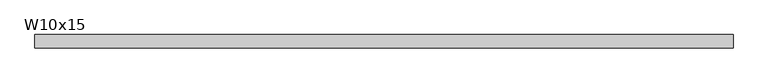
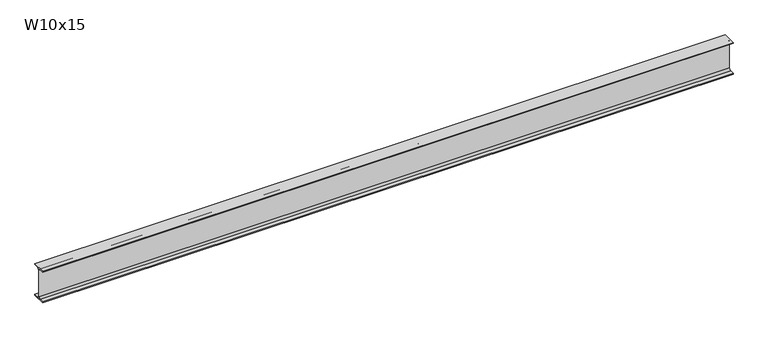
"""IFC4 building model written with IfcOpenShell, lengths in millimetres: beam geometry, RME W-Wide Flange : W10x15."""

from ifc_helpers import new_model, si_unit, point, frame, frame_2d, origin, place, context, project, spatial, polyline, circle_curve, trimmed, segment, composite_curve, outline, extrude, source, transform, mapped, element, save


def w10x15_b66c4662(model_context):
    return source(origin(), model_context, "Body", "SweptSolid", [
        extrude(outline(composite_curve([segment(polyline([(50.8, -120.142), (50.8, -127.0), (-50.8, -127.0), (-50.8, -120.142), (-16.7005, -120.142)]), True, "CONTINUOUS"), segment(trimmed(circle_curve(frame_2d((-16.7005, -106.3625)), 13.7795), [point((-16.7005, -120.142))], [point((-2.921, -106.3625))], True, "CARTESIAN"), True, "CONTINUOUS"), segment(polyline([(-2.921, -106.3625), (-2.921, 106.3625)]), True, "CONTINUOUS"), segment(trimmed(circle_curve(frame_2d((-16.7005, 106.3625)), 13.7795), [point((-2.921, 106.3625))], [point((-16.7005, 120.142))], True, "CARTESIAN"), True, "CONTINUOUS"), segment(polyline([(-16.7005, 120.142), (-50.8, 120.142), (-50.8, 127.0), (50.8, 127.0), (50.8, 120.142), (16.7005, 120.142)]), True, "CONTINUOUS"), segment(trimmed(circle_curve(frame_2d((16.7005, 106.3625)), 13.7795), [point((16.7005, 120.142))], [point((2.921, 106.3625))], True, "CARTESIAN"), True, "CONTINUOUS"), segment(polyline([(2.921, 106.3625), (2.921, -106.3625)]), True, "CONTINUOUS"), segment(trimmed(circle_curve(frame_2d((16.7005, -106.3625)), 13.7795), [point((2.921, -106.3625))], [point((16.7005, -120.142))], True, "CARTESIAN"), True, "CONTINUOUS"), segment(polyline([(16.7005, -120.142), (50.8, -120.142)]), True, "CONTINUOUS")], self_intersect=False)), frame((-2628.8886716, 0.0, 0.0), z_axis=(1.0, 0.0, 0.0), x_axis=(0.0, 1.0, 0.0)), (0.0, 0.0, 1.0), 5257.7773433),
    ])


if __name__ == "__main__":
    model = new_model("IFC4")
    model_context = context("Model", 3, world=origin())
    ifc_project = project(units=[si_unit("LENGTHUNIT", "METRE", prefix="MILLI")], contexts=[model_context])
    site = spatial("IfcSite", under=ifc_project)
    building = spatial("IfcBuilding", under=site)
    placement = place(None, origin())
    w10x15_shape = w10x15_b66c4662(model_context)
    element("IfcBeam", 1, ObjectType="RME W-Wide Flange : W10x15", at=placement, inside=building, context=model_context, shape_type="MappedRepresentation", body=[
        mapped(w10x15_shape, transform((0.0, 0.0, 0.0), x_axis=(1.0, 0.0, 0.0), y_axis=(0.0, 1.0, 0.0), z_axis=(0.0, 0.0, 1.0))),
    ])
    save(model, "model.ifc")

# Revit data of these elements
# Type "RME W-Wide Flange : W10x15"
#   WELD P [instance default] = ""
#   WELD LE [instance default] = ""
#   WELD D [instance default] = ""
#   TOP SECTION SIZE [instance default] = ""
#   TOP SECTION LENGTH [instance default] = ""
#   REMARKS [instance default] = ""
#   REINF TYPE [instance default] = ""
#   Nominal Size = "W24"
#   End Bearing Capacity [instance default] = ""
#   BOT SECTION SIZE [instance default] = ""
#   BOT SECTION LENGTH [instance default] = ""
#   Assembly Code = "B10"
#   W = 15
#   Start Extension Calculation [instance default] = 10' - 0"
#   Start Extension [instance default] = -0' - 0 1/2"
#   End Extension Calculation [instance default] = 10' - 0"
#   End Extension [instance default] = -0' - 0 1/2"
#   Length [instance default] = 5' - 0"
#   bf = 0' - 4"
#   d = 0' - 10"
#   k = 0' - 0 13/16"
#   k2 = 0' - 0.5425"
#   tf = 0' - 0.27"
#   tw = 0' - 0.23"
#   A = 0.030625 SF
#   Structural Material [instance default] = Metal - Steel - ASTM A992
# Element 1 (IfcBeam, "RME W-Wide Flange : W10x15")
#   Length = 17' - 2.99911"
#   Materials on its faces: "Metal - Steel - ASTM A992"
# Materials
#   "Metal - Steel - ASTM A992": class "Metal", colour RGB 255 128 0, transparency 0
